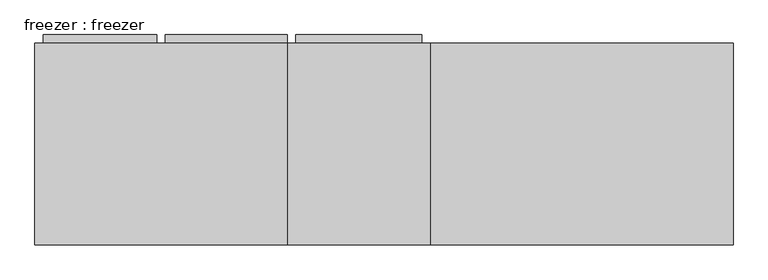
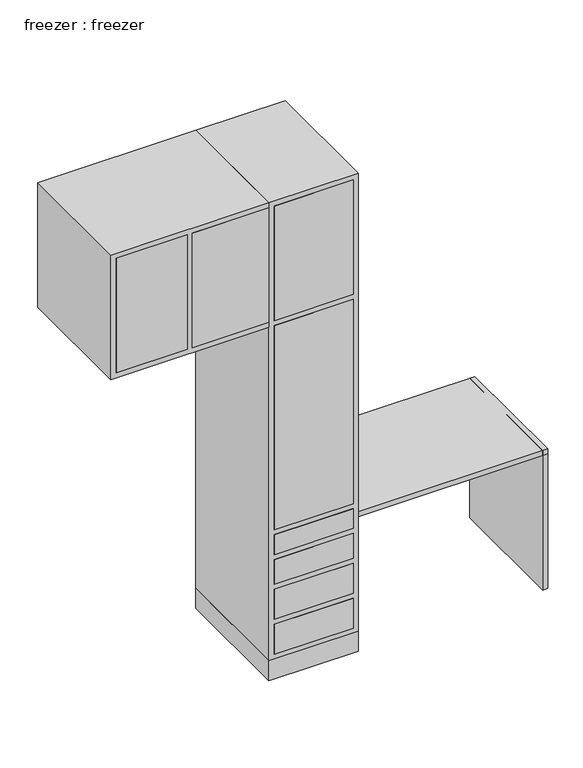
"""IFC4 building model written with IfcOpenShell, lengths in millimetres: proxy geometry, freezer : freezer."""

from ifc_helpers import new_model, si_unit, frame, origin, place, context, project, spatial, polyline, outline, extrude, source, transform, mapped, element, save


def freezer_freezer_4e8b300b(model_context):
    return source(origin(), model_context, "Body", "SweptSolid", [
        extrude(outline(polyline([(-800.1, 685.8), (-431.8, 685.8), (-431.8, 50.8), (-800.1, 50.8), (-800.1, 685.8)])), frame((0.0, 0.0, 2542.2131475), z_axis=(0.0, 0.0, 1.0), x_axis=(1.0, 0.0, 0.0)), (0.0, 0.0, 1.0), 584.2),
        extrude(outline(polyline([(-1168.4, 685.8), (-825.5, 685.8), (-825.5, 50.8), (-1168.4, 50.8), (-1168.4, 685.8)])), frame((0.0, 0.0, 2542.2131475), z_axis=(0.0, 0.0, 1.0), x_axis=(1.0, 0.0, 0.0)), (0.0, 0.0, 1.0), 584.2),
        extrude(outline(polyline([(-1193.8, 660.4), (-431.8, 660.4), (-431.8, 50.8), (-1193.8, 50.8), (-1193.8, 660.4)])), frame((0.0, 0.0, 2516.8131475), z_axis=(0.0, 0.0, 1.0), x_axis=(1.0, 0.0, 0.0)), (0.0, 0.0, 1.0), 635.0),
        extrude(outline(polyline([(-406.4, 685.8), (-25.4, 685.8), (-25.4, 50.8), (-406.4, 50.8), (-406.4, 685.8)])), frame((0.0, 0.0, 2542.2131475), z_axis=(0.0, 0.0, 1.0), x_axis=(1.0, 0.0, 0.0)), (0.0, 0.0, 1.0), 584.2),
        extrude(outline(polyline([(-406.4, 685.8), (-25.4, 685.8), (-25.4, 50.8), (-406.4, 50.8), (-406.4, 685.8)])), frame((0.0, 0.0, 1475.4131475), z_axis=(0.0, 0.0, 1.0), x_axis=(1.0, 0.0, 0.0)), (0.0, 0.0, 1.0), 1041.4),
        extrude(outline(polyline([(-406.4, 685.8), (-25.4, 685.8), (-25.4, 50.8), (-406.4, 50.8), (-406.4, 685.8)])), frame((0.0, 0.0, 1348.4131475), z_axis=(0.0, 0.0, 1.0), x_axis=(1.0, 0.0, 0.0)), (0.0, 0.0, 1.0), 101.6),
        extrude(outline(polyline([(-406.4, 685.8), (-25.4, 685.8), (-25.4, 50.8), (-406.4, 50.8), (-406.4, 685.8)])), frame((0.0, 0.0, 1196.0131475), z_axis=(0.0, 0.0, 1.0), x_axis=(1.0, 0.0, 0.0)), (0.0, 0.0, 1.0), 127.0),
        extrude(outline(polyline([(-406.4, 685.8), (-25.4, 685.8), (-25.4, 50.8), (-406.4, 50.8), (-406.4, 685.8)])), frame((0.0, 0.0, 1018.2131475), z_axis=(0.0, 0.0, 1.0), x_axis=(1.0, 0.0, 0.0)), (0.0, 0.0, 1.0), 152.4),
        extrude(outline(polyline([(-406.4, 685.8), (-25.4, 685.8), (-25.4, 50.8), (-406.4, 50.8), (-406.4, 685.8)])), frame((0.0, 0.0, 840.4131475), z_axis=(0.0, 0.0, 1.0), x_axis=(1.0, 0.0, 0.0)), (0.0, 0.0, 1.0), 152.4),
        extrude(outline(polyline([(-431.8, 660.4), (0.0, 660.4), (0.0, 50.8), (-431.8, 50.8), (-431.8, 660.4)])), frame((0.0, 0.0, 713.4131475), z_axis=(0.0, 0.0, 1.0), x_axis=(1.0, 0.0, 0.0)), (0.0, 0.0, 1.0), 101.6),
        extrude(outline(polyline([(-431.8, 660.4), (0.0, 660.4), (0.0, 50.8), (-431.8, 50.8), (-431.8, 660.4)])), frame((0.0, 0.0, 713.4131475), z_axis=(0.0, 0.0, 1.0), x_axis=(1.0, 0.0, 0.0)), (0.0, 0.0, 1.0), 2438.4),
        extrude(outline(polyline([(0.0, 660.4), (914.4, 660.4), (914.4, 50.8), (0.0, 50.8), (0.0, 660.4)])), frame((0.0, 0.0, 1399.2131475), z_axis=(0.0, 0.0, 1.0), x_axis=(1.0, 0.0, 0.0)), (0.0, 0.0, 1.0), 25.4),
        extrude(outline(polyline([(889.0, 660.4), (914.4, 660.4), (914.4, 50.8), (889.0, 50.8), (889.0, 660.4)])), frame((0.0, 0.0, 713.4131475), z_axis=(0.0, 0.0, 1.0), x_axis=(1.0, 0.0, 0.0)), (0.0, 0.0, 1.0), 711.2),
    ])


if __name__ == "__main__":
    model = new_model("IFC4")
    model_context = context("Model", 3, world=origin())
    ifc_project = project(units=[si_unit("LENGTHUNIT", "METRE", prefix="MILLI")], contexts=[model_context])
    site = spatial("IfcSite", under=ifc_project)
    building = spatial("IfcBuilding", under=site)
    placement = place(None, origin())
    freezer_freezer_shape = freezer_freezer_4e8b300b(model_context)
    element("IfcBuildingElementProxy", 1, Name="freezer : freezer", ObjectType="freezer : freezer", at=placement, inside=building, context=model_context, shape_type="MappedRepresentation", body=[
        mapped(freezer_freezer_shape, transform((0.0, 0.0, 0.0), x_axis=(1.0, 0.0, 0.0), y_axis=(0.0, 1.0, 0.0), z_axis=(0.0, 0.0, 1.0))),
    ])
    save(model, "model.ifc")

# Revit data of these elements
# Type "freezer : freezer"
#   drawer depth = 2' - 1"
#   cabinet depth = 2' - 0"
#   Default Elevation = 0
